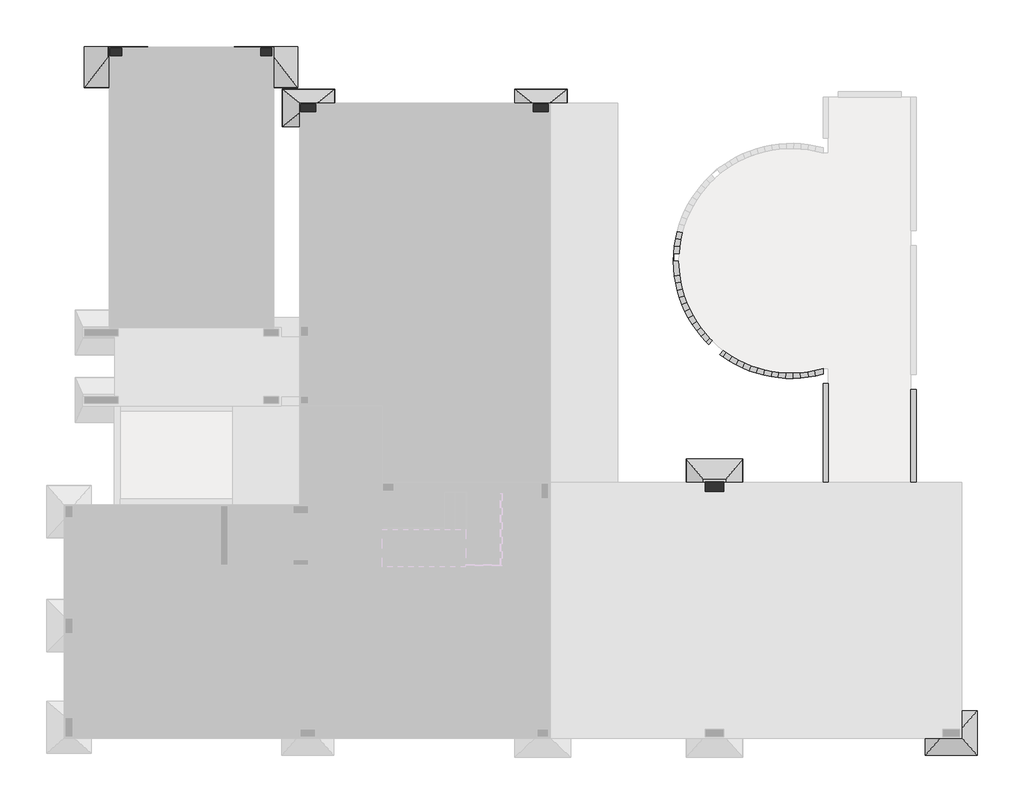
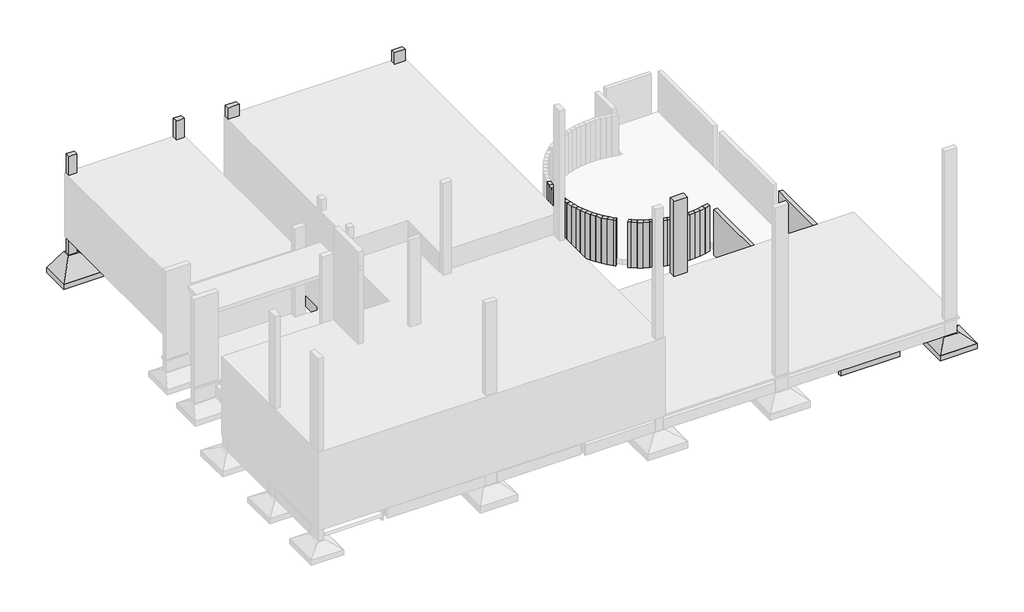
# One storey, part 3 of 4: 37 beams, 7 fasteners, 5 columns.
# Revit data of these elements (continued)
# Type "TQS - Sapata : S13" (continued)
#   EXCXABS = 0.75 m
#   EXCX = 0.00 m
#   DIMY = 1.50 m
#   DIMX = 1.50 m
#   Material estrutural = Concreto - Concreto concretado no local
#   Width = 0
#   Length = 0
# Type "TQS - Sapata : S2"
#   TY = 0.40 m
#   TX = 0.29 m
#   HS = 0.60 m
#   H0 = 0.20 m
#   EXCYABS = 0.85 m
#   EXCY = 0.00 m
#   EXCXABS = 0.145 m
#   EXCX = -0.405 m
#   DIMY = 1.70 m
#   DIMX = 1.10 m
#   Material estrutural = Concreto - Concreto concretado no local
#   Width = 0
#   Length = 0
# Type "TQS - Sapata : S24"
#   TY = 0.60 m
#   TX = 0.29 m
#   HS = 0.50 m
#   H0 = 0.20 m
#   EXCYABS = 0.70 m
#   EXCY = 0.00 m
#   EXCXABS = 0.60 m
#   EXCX = 0.00 m
#   DIMY = 1.40 m
#   DIMX = 1.20 m
#   Material estrutural = Concreto - Concreto concretado no local
#   Width = 0
#   Length = 0
# Type "TQS - Sapata : S3"
#   TY = 0.50 m
#   TX = 0.29 m
#   HS = 0.50 m
#   H0 = 0.20 m
#   EXCYABS = 0.70 m
#   EXCY = 0.00 m
#   EXCXABS = 0.50 m
#   EXCX = 0.00 m
#   DIMY = 1.40 m
#   DIMX = 1.00 m
#   Material estrutural = Concreto - Concreto concretado no local
#   Width = 0
#   Length = 0
# Type "TQS - Sapata : S4"
#   TY = 0.50 m
#   TX = 0.29 m
#   HS = 0.50 m
#   H0 = 0.20 m
#   EXCYABS = 0.70 m
#   EXCY = 0.00 m
#   EXCXABS = 0.50 m
#   EXCX = 0.00 m
#   DIMY = 1.40 m
#   DIMX = 1.00 m
#   Material estrutural = Concreto - Concreto concretado no local
#   Width = 0
#   Length = 0
# Element 1 (IfcBeam, "TQS - Viga retangular : 14.0 x 180.0")
#   Uso = "ESTRUTURA"
#   Titulo = "VP2"
#   Chave = "-984"
#   Tipo Elemento = "Viga"
#   SHA1 = "67BB47F7F07D141E1E461B1B62FFCED57BE49A5E"
#   Revisão = ""
#   Tipo de carga = ""
#   Divisor de flexao = ""
#   Secao = ""
#   Configuracao = ""
#   Angulo (graus) = ""
#   Detalhamento = ""
#   Casos de vento manual = ""
#   Tipo = ""
#   Alcas = ""
#   Furos = ""
#   Pino = ""
#   Distribuicao = ""
#   Solidarizado = ""
#   Solidarizar na montagem = ""
#   Unir com o próximo = ""
#   Grupo pre moldado = ""
#   Verificado = ""
#   Concreto C = ""
#   Taxa de armadura (kgf/m³) = 0
#   Carga (tf/m²) = 0
#   Carga (tf/m) = 0
#   Carga (tf) = 0
#   Altura = 1.80 m
#   Rebaixo = 0.15 m
#   Largura = 0.14 m
#   Distancia a face = 0.00 m
#   Distancia ao eixo = 0.00 m
#   Altura gerber esquerda = 0.00 m
#   Largura gerber esquerda = 0.00 m
#   Altura gerber direita = 0.00 m
#   Largura gerber direita = 0.00 m
#   Resultado de Ensaios fck (MPa) = 0
#   Unique TQS ID = -984
#   Principal = yes
#   Structural Material = none
#   Phase Created = CC_AP/ESTR
# Element 2 (IfcBeam, "TQS - Viga retangular : 14.0 x 180.0")
#   Uso = "ESTRUTURA"
#   Titulo = "VP3"
#   Chave = "-985"
#   Tipo Elemento = "Viga"
#   SHA1 = "1D3F2A738C11C779DD3B877E14C8E10A324E012C"
#   Revisão = ""
#   Tipo de carga = ""
#   Divisor de flexao = ""
#   Secao = ""
#   Configuracao = ""
#   Angulo (graus) = ""
#   Detalhamento = ""
#   Casos de vento manual = ""
#   Tipo = ""
#   Alcas = ""
#   Furos = ""
#   Pino = ""
#   Distribuicao = ""
#   Solidarizado = ""
#   Solidarizar na montagem = ""
#   Unir com o próximo = ""
#   Grupo pre moldado = ""
#   Verificado = ""
#   Concreto C = ""
#   Taxa de armadura (kgf/m³) = 0
#   Carga (tf/m²) = 0
#   Carga (tf/m) = 0
#   Carga (tf) = 0
#   Altura = 1.80 m
#   Rebaixo = 0.15 m
#   Largura = 0.14 m
#   Distancia a face = 0.00 m
#   Distancia ao eixo = 0.00 m
#   Altura gerber esquerda = 0.00 m
#   Largura gerber esquerda = 0.00 m
#   Altura gerber direita = 0.00 m
#   Largura gerber direita = 0.00 m
#   Resultado de Ensaios fck (MPa) = 0
#   Unique TQS ID = -985
#   Principal = yes
#   Structural Material = none
#   Phase Created = CC_AP/ESTR
# Element 3 (IfcBeam, "TQS - Viga retangular : 14.0 x 180.0")
#   Uso = "ESTRUTURA"
#   Titulo = "VP4"
#   Chave = "-987"
#   Tipo Elemento = "Viga"
#   SHA1 = "18E803970E3FF61AE3A7C4B8095E8E40226C0AA9"
#   Revisão = ""
#   Tipo de carga = ""
#   Divisor de flexao = ""
#   Secao = ""
#   Configuracao = ""
#   Angulo (graus) = ""
#   Detalhamento = ""
#   Casos de vento manual = ""
#   Tipo = ""
#   Alcas = ""
#   Furos = ""
#   Pino = ""
#   Distribuicao = ""
#   Solidarizado = ""
#   Solidarizar na montagem = ""
#   Unir com o próximo = ""
#   Grupo pre moldado = ""
#   Verificado = ""
#   Concreto C = ""
#   Taxa de armadura (kgf/m³) = 0
#   Carga (tf/m²) = 0
#   Carga (tf/m) = 0
#   Carga (tf) = 0
#   Altura = 1.80 m
#   Rebaixo = 0.15 m
#   Largura = 0.14 m
#   Distancia a face = 0.00 m
#   Distancia ao eixo = 0.00 m
#   Altura gerber esquerda = 0.00 m
#   Largura gerber esquerda = 0.00 m
#   Altura gerber direita = 0.00 m
#   Largura gerber direita = 0.00 m
#   Resultado de Ensaios fck (MPa) = 0
#   Unique TQS ID = -987
#   Principal = yes
#   Structural Material = none
#   Phase Created = CC_AP/ESTR
# Element 4 (IfcBeam, "TQS - Viga retangular : 14.0 x 180.0")
#   Uso = "ESTRUTURA"
#   Titulo = "VP4"
#   Chave = "-988"
#   Tipo Elemento = "Viga"
#   SHA1 = "B71FF30D7224BC3A2F9C0912C04A339394FFFF18"
#   Revisão = ""
#   Tipo de carga = ""
#   Divisor de flexao = ""
#   Secao = ""
#   Configuracao = ""
#   Angulo (graus) = ""
#   Detalhamento = ""
#   Casos de vento manual = ""
#   Tipo = ""
#   Alcas = ""
#   Furos = ""
#   Pino = ""
#   Distribuicao = ""
#   Solidarizado = ""
#   Solidarizar na montagem = ""
#   Unir com o próximo = ""
#   Grupo pre moldado = ""
#   Verificado = ""
#   Concreto C = ""
#   Taxa de armadura (kgf/m³) = 0
#   Carga (tf/m²) = 0
#   Carga (tf/m) = 0
#   Carga (tf) = 0
#   Altura = 1.80 m
#   Rebaixo = 0.15 m
#   Largura = 0.14 m
#   Distancia a face = 0.00 m
#   Distancia ao eixo = 0.00 m
#   Altura gerber esquerda = 0.00 m
#   Largura gerber esquerda = 0.00 m
#   Altura gerber direita = 0.00 m
#   Largura gerber direita = 0.00 m
#   Resultado de Ensaios fck (MPa) = 0
#   Unique TQS ID = -988
#   Principal = yes
#   Structural Material = none
#   Phase Created = CC_AP/ESTR
# Element 5 (IfcBeam, "TQS - Viga retangular : 14.0 x 180.0")
#   Uso = "ESTRUTURA"
#   Titulo = "VP4"
#   Chave = "-989"
#   Tipo Elemento = "Viga"
#   SHA1 = "E9E1B2FEFAB6FC9E808C50FA3A91823AD53CDAD9"
#   Revisão = ""
#   Tipo de carga = ""
#   Divisor de flexao = ""
#   Secao = ""
#   Configuracao = ""
#   Angulo (graus) = ""
#   Detalhamento = ""
#   Casos de vento manual = ""
#   Tipo = ""
#   Alcas = ""
#   Furos = ""
#   Pino = ""
#   Distribuicao = ""
#   Solidarizado = ""
#   Solidarizar na montagem = ""
#   Unir com o próximo = ""
#   Grupo pre moldado = ""
#   Verificado = ""
#   Concreto C = ""
#   Taxa de armadura (kgf/m³) = 0
#   Carga (tf/m²) = 0
#   Carga (tf/m) = 0
#   Carga (tf) = 0
#   Altura = 1.80 m
#   Rebaixo = 0.15 m
#   Largura = 0.14 m
#   Distancia a face = 0.00 m
#   Distancia ao eixo = 0.00 m
#   Altura gerber esquerda = 0.00 m
#   Largura gerber esquerda = 0.00 m
#   Altura gerber direita = 0.00 m
#   Largura gerber direita = 0.00 m
#   Resultado de Ensaios fck (MPa) = 0
#   Unique TQS ID = -989
#   Principal = yes
#   Structural Material = none
#   Phase Created = CC_AP/ESTR
# Element 6 (IfcBeam, "TQS - Viga retangular : 14.0 x 180.0")
#   Uso = "ESTRUTURA"
#   Titulo = "VP4"
#   Chave = "-990"
#   Tipo Elemento = "Viga"
#   SHA1 = "A4F79934EF83F3B7E9A1E2CD35D009C4681F812D"
#   Revisão = ""
#   Tipo de carga = ""
#   Divisor de flexao = ""
#   Secao = ""
#   Configuracao = ""
#   Angulo (graus) = ""
#   Detalhamento = ""
#   Casos de vento manual = ""
#   Tipo = ""
#   Alcas = ""
#   Furos = ""
#   Pino = ""
#   Distribuicao = ""
#   Solidarizado = ""
#   Solidarizar na montagem = ""
#   Unir com o próximo = ""
#   Grupo pre moldado = ""
#   Verificado = ""
#   Concreto C = ""
#   Taxa de armadura (kgf/m³) = 0
#   Carga (tf/m²) = 0
#   Carga (tf/m) = 0
#   Carga (tf) = 0
#   Altura = 1.80 m
#   Rebaixo = 0.15 m
#   Largura = 0.14 m
#   Distancia a face = 0.00 m
#   Distancia ao eixo = 0.00 m
#   Altura gerber esquerda = 0.00 m
#   Largura gerber esquerda = 0.00 m
#   Altura gerber direita = 0.00 m
#   Largura gerber direita = 0.00 m
#   Resultado de Ensaios fck (MPa) = 0
#   Unique TQS ID = -990
#   Principal = yes
#   Structural Material = none
#   Phase Created = CC_AP/ESTR
# Element 7 (IfcBeam, "TQS - Viga retangular : 14.0 x 180.0")
#   Uso = "ESTRUTURA"
#   Titulo = "VP4"
#   Chave = "-991"
#   Tipo Elemento = "Viga"
#   SHA1 = "59C2882C15F8D77C9BC823B17A9B229971BFE292"
#   Revisão = ""
#   Tipo de carga = ""
#   Divisor de flexao = ""
#   Secao = ""
#   Configuracao = ""
#   Angulo (graus) = ""
#   Detalhamento = ""
#   Casos de vento manual = ""
#   Tipo = ""
#   Alcas = ""
#   Furos = ""
#   Pino = ""
#   Distribuicao = ""
#   Solidarizado = ""
#   Solidarizar na montagem = ""
#   Unir com o próximo = ""
#   Grupo pre moldado = ""
#   Verificado = ""
#   Concreto C = ""
#   Taxa de armadura (kgf/m³) = 0
#   Carga (tf/m²) = 0
#   Carga (tf/m) = 0
#   Carga (tf) = 0
#   Altura = 1.80 m
#   Rebaixo = 0.15 m
#   Largura = 0.14 m
#   Distancia a face = 0.00 m
#   Distancia ao eixo = 0.00 m
#   Altura gerber esquerda = 0.00 m
#   Largura gerber esquerda = 0.00 m
#   Altura gerber direita = 0.00 m
#   Largura gerber direita = 0.00 m
#   Resultado de Ensaios fck (MPa) = 0
#   Unique TQS ID = -991
#   Principal = yes
#   Structural Material = none
#   Phase Created = CC_AP/ESTR
# Element 8 (IfcBeam, "TQS - Viga retangular : 14.0 x 180.0")
#   Uso = "ESTRUTURA"
#   Titulo = "VP4"
#   Chave = "-992"
#   Tipo Elemento = "Viga"
#   SHA1 = "6D985E6B9F5FA1FD140F505980BE925AA5C487F2"
#   Revisão = ""
#   Tipo de carga = ""
#   Divisor de flexao = ""
#   Secao = ""
#   Configuracao = ""
#   Angulo (graus) = ""
#   Detalhamento = ""
#   Casos de vento manual = ""
#   Tipo = ""
#   Alcas = ""
#   Furos = ""
#   Pino = ""
#   Distribuicao = ""
#   Solidarizado = ""
#   Solidarizar na montagem = ""
#   Unir com o próximo = ""
#   Grupo pre moldado = ""
#   Verificado = ""
#   Concreto C = ""
#   Taxa de armadura (kgf/m³) = 0
#   Carga (tf/m²) = 0
#   Carga (tf/m) = 0
#   Carga (tf) = 0
#   Altura = 1.80 m
#   Rebaixo = 0.15 m
#   Largura = 0.14 m
#   Distancia a face = 0.00 m
#   Distancia ao eixo = 0.00 m
#   Altura gerber esquerda = 0.00 m
#   Largura gerber esquerda = 0.00 m
#   Altura gerber direita = 0.00 m
#   Largura gerber direita = 0.00 m
#   Resultado de Ensaios fck (MPa) = 0
#   Unique TQS ID = -992
#   Principal = yes
#   Structural Material = none
#   Phase Created = CC_AP/ESTR
# Element 9 (IfcBeam, "TQS - Viga retangular : 14.0 x 180.0")
#   Uso = "ESTRUTURA"
#   Titulo = "VP4"
#   Chave = "-993"
#   Tipo Elemento = "Viga"
#   SHA1 = "5D4E92287FB362FDFCD64B2B7E6C35302CB92A79"
#   Revisão = ""
#   Tipo de carga = ""
#   Divisor de flexao = ""
#   Secao = ""
#   Configuracao = ""
#   Angulo (graus) = ""
#   Detalhamento = ""
#   Casos de vento manual = ""
#   Tipo = ""
#   Alcas = ""
#   Furos = ""
#   Pino = ""
#   Distribuicao = ""
#   Solidarizado = ""
#   Solidarizar na montagem = ""
#   Unir com o próximo = ""
#   Grupo pre moldado = ""
#   Verificado = ""
#   Concreto C = ""
#   Taxa de armadura (kgf/m³) = 0
#   Carga (tf/m²) = 0
#   Carga (tf/m) = 0
#   Carga (tf) = 0
#   Altura = 1.80 m
#   Rebaixo = 0.15 m
#   Largura = 0.14 m
#   Distancia a face = 0.00 m
#   Distancia ao eixo = 0.00 m
#   Altura gerber esquerda = 0.00 m
#   Largura gerber esquerda = 0.00 m
#   Altura gerber direita = 0.00 m
#   Largura gerber direita = 0.00 m
#   Resultado de Ensaios fck (MPa) = 0
#   Unique TQS ID = -993
#   Principal = yes
#   Structural Material = none
#   Phase Created = CC_AP/ESTR
# Element 10 (IfcBeam, "TQS - Viga retangular : 14.0 x 180.0")
#   Uso = "ESTRUTURA"
#   Titulo = "VP4"
#   Chave = "-994"
#   Tipo Elemento = "Viga"
#   SHA1 = "B241F61C6536B176DF9E3A8727FE075D16BE7057"
#   Revisão = ""
#   Tipo de carga = ""
#   Divisor de flexao = ""
#   Secao = ""
#   Configuracao = ""
#   Angulo (graus) = ""
#   Detalhamento = ""
#   Casos de vento manual = ""
#   Tipo = ""
#   Alcas = ""
#   Furos = ""
#   Pino = ""
#   Distribuicao = ""
#   Solidarizado = ""
#   Solidarizar na montagem = ""
#   Unir com o próximo = ""
#   Grupo pre moldado = ""
#   Verificado = ""
#   Concreto C = ""
#   Taxa de armadura (kgf/m³) = 0
#   Carga (tf/m²) = 0
#   Carga (tf/m) = 0
#   Carga (tf) = 0
#   Altura = 1.80 m
#   Rebaixo = 0.15 m
#   Largura = 0.14 m
#   Distancia a face = 0.00 m
#   Distancia ao eixo = 0.00 m
#   Altura gerber esquerda = 0.00 m
#   Largura gerber esquerda = 0.00 m
#   Altura gerber direita = 0.00 m
#   Largura gerber direita = 0.00 m
#   Resultado de Ensaios fck (MPa) = 0
#   Unique TQS ID = -994
#   Principal = yes
#   Structural Material = none
#   Phase Created = CC_AP/ESTR
# Element 11 (IfcBeam, "TQS - Viga retangular : 14.0 x 180.0")
#   Uso = "ESTRUTURA"
#   Titulo = "VP4"
#   Chave = "-995"
#   Tipo Elemento = "Viga"
#   SHA1 = "79F2E8F443EC2E8CC5B8F506A3E5025E7F953CE7"
#   Revisão = ""
#   Tipo de carga = ""
#   Divisor de flexao = ""
#   Secao = ""
#   Configuracao = ""
#   Angulo (graus) = ""
#   Detalhamento = ""
#   Casos de vento manual = ""
#   Tipo = ""
#   Alcas = ""
#   Furos = ""
#   Pino = ""
#   Distribuicao = ""
#   Solidarizado = ""
#   Solidarizar na montagem = ""
#   Unir com o próximo = ""
#   Grupo pre moldado = ""
#   Verificado = ""
#   Concreto C = ""
#   Taxa de armadura (kgf/m³) = 0
#   Carga (tf/m²) = 0
#   Carga (tf/m) = 0
#   Carga (tf) = 0
#   Altura = 1.80 m
#   Rebaixo = 0.15 m
#   Largura = 0.14 m
#   Distancia a face = 0.00 m
#   Distancia ao eixo = 0.00 m
#   Altura gerber esquerda = 0.00 m
#   Largura gerber esquerda = 0.00 m
#   Altura gerber direita = 0.00 m
#   Largura gerber direita = 0.00 m
#   Resultado de Ensaios fck (MPa) = 0
#   Unique TQS ID = -995
#   Principal = yes
#   Structural Material = none
#   Phase Created = CC_AP/ESTR
# Element 12 (IfcBeam, "TQS - Viga retangular : 14.0 x 180.0")
#   Uso = "ESTRUTURA"
#   Titulo = "VP4"
#   Chave = "-996"
#   Tipo Elemento = "Viga"
#   SHA1 = "EC69CF733B6B75DD72A616518C986B1D4EC6373A"
#   Revisão = ""
#   Tipo de carga = ""
#   Divisor de flexao = ""
#   Secao = ""
#   Configuracao = ""
#   Angulo (graus) = ""
#   Detalhamento = ""
#   Casos de vento manual = ""
#   Tipo = ""
#   Alcas = ""
#   Furos = ""
#   Pino = ""
#   Distribuicao = ""
#   Solidarizado = ""
#   Solidarizar na montagem = ""
#   Unir com o próximo = ""
#   Grupo pre moldado = ""
#   Verificado = ""
#   Concreto C = ""
#   Taxa de armadura (kgf/m³) = 0
#   Carga (tf/m²) = 0
#   Carga (tf/m) = 0
#   Carga (tf) = 0
#   Altura = 1.80 m
#   Rebaixo = 0.15 m
#   Largura = 0.14 m
#   Distancia a face = 0.00 m
#   Distancia ao eixo = 0.00 m
#   Altura gerber esquerda = 0.00 m
#   Largura gerber esquerda = 0.00 m
#   Altura gerber direita = 0.00 m
#   Largura gerber direita = 0.00 m
#   Resultado de Ensaios fck (MPa) = 0
#   Unique TQS ID = -996
#   Principal = yes
#   Structural Material = none
#   Phase Created = CC_AP/ESTR
# Element 13 (IfcBeam, "TQS - Viga retangular : 14.0 x 180.0")
#   Uso = "ESTRUTURA"
#   Titulo = "VP4"
#   Chave = "-997"
#   Tipo Elemento = "Viga"
#   SHA1 = "A94BB0AB94C95055560F49AF3BCE408F9E38B8C0"
#   Revisão = ""
#   Tipo de carga = ""
#   Divisor de flexao = ""
#   Secao = ""
#   Configuracao = ""
#   Angulo (graus) = ""
#   Detalhamento = ""
#   Casos de vento manual = ""
#   Tipo = ""
#   Alcas = ""
#   Furos = ""
#   Pino = ""
#   Distribuicao = ""
#   Solidarizado = ""
#   Solidarizar na montagem = ""
#   Unir com o próximo = ""
#   Grupo pre moldado = ""
#   Verificado = ""
#   Concreto C = ""
#   Taxa de armadura (kgf/m³) = 0
#   Carga (tf/m²) = 0
#   Carga (tf/m) = 0
#   Carga (tf) = 0
#   Altura = 1.80 m
#   Rebaixo = 0.15 m
#   Largura = 0.14 m
#   Distancia a face = 0.00 m
#   Distancia ao eixo = 0.00 m
#   Altura gerber esquerda = 0.00 m
#   Largura gerber esquerda = 0.00 m
#   Altura gerber direita = 0.00 m
#   Largura gerber direita = 0.00 m
#   Resultado de Ensaios fck (MPa) = 0
#   Unique TQS ID = -997
#   Principal = yes
#   Structural Material = none
#   Phase Created = CC_AP/ESTR
# Element 14 (IfcBeam, "TQS - Viga retangular : 14.0 x 180.0")
#   Uso = "ESTRUTURA"
#   Titulo = "VP4"
#   Chave = "-998"
#   Tipo Elemento = "Viga"
#   SHA1 = "6378FB8D39603434150BF0AD569D703CFB80FE5F"
#   Revisão = ""
#   Tipo de carga = ""
#   Divisor de flexao = ""
#   Secao = ""
#   Configuracao = ""
#   Angulo (graus) = ""
#   Detalhamento = ""
#   Casos de vento manual = ""
#   Tipo = ""
#   Alcas = ""
#   Furos = ""
#   Pino = ""
#   Distribuicao = ""
#   Solidarizado = ""
#   Solidarizar na montagem = ""
#   Unir com o próximo = ""
#   Grupo pre moldado = ""
#   Verificado = ""
#   Concreto C = ""
#   Taxa de armadura (kgf/m³) = 0
#   Carga (tf/m²) = 0
#   Carga (tf/m) = 0
#   Carga (tf) = 0
#   Altura = 1.80 m
#   Rebaixo = 0.15 m
#   Largura = 0.14 m
#   Distancia a face = 0.00 m
#   Distancia ao eixo = 0.00 m
#   Altura gerber esquerda = 0.00 m
#   Largura gerber esquerda = 0.00 m
#   Altura gerber direita = 0.00 m
#   Largura gerber direita = 0.00 m
#   Resultado de Ensaios fck (MPa) = 0
#   Unique TQS ID = -998
#   Principal = yes
#   Structural Material = none
#   Phase Created = CC_AP/ESTR
# Element 15 (IfcBeam, "TQS - Viga retangular : 14.0 x 180.0")
#   Uso = "ESTRUTURA"
#   Titulo = "VP4"
#   Chave = "-999"
#   Tipo Elemento = "Viga"
#   SHA1 = "2B4C78D211D826E735DAAC0C825AB5B97130EBCE"
#   Revisão = ""
#   Tipo de carga = ""
#   Divisor de flexao = ""
#   Secao = ""
#   Configuracao = ""
#   Angulo (graus) = ""
#   Detalhamento = ""
#   Casos de vento manual = ""
#   Tipo = ""
#   Alcas = ""
#   Furos = ""
#   Pino = ""
#   Distribuicao = ""
#   Solidarizado = ""
#   Solidarizar na montagem = ""
#   Unir com o próximo = ""
#   Grupo pre moldado = ""
#   Verificado = ""
#   Concreto C = ""
#   Taxa de armadura (kgf/m³) = 0
#   Carga (tf/m²) = 0
#   Carga (tf/m) = 0
#   Carga (tf) = 0
#   Altura = 1.80 m
#   Rebaixo = 0.15 m
#   Largura = 0.14 m
#   Distancia a face = 0.00 m
#   Distancia ao eixo = 0.00 m
#   Altura gerber esquerda = 0.00 m
#   Largura gerber esquerda = 0.00 m
#   Altura gerber direita = 0.00 m
#   Largura gerber direita = 0.00 m
#   Resultado de Ensaios fck (MPa) = 0
#   Unique TQS ID = -999
#   Principal = yes
#   Structural Material = none
#   Phase Created = CC_AP/ESTR
# Element 16 (IfcBeam, "TQS - Viga retangular : 14.0 x 180.0")
#   Uso = "ESTRUTURA"
#   Titulo = "VP4"
#   Chave = "-1000"
#   Tipo Elemento = "Viga"
#   SHA1 = "DD50D292EAFD20D7EF85643CCD075ACF91033CA0"
#   Revisão = ""
#   Tipo de carga = ""
#   Divisor de flexao = ""
#   Secao = ""
#   Configuracao = ""
#   Angulo (graus) = ""
#   Detalhamento = ""
#   Casos de vento manual = ""
#   Tipo = ""
#   Alcas = ""
#   Furos = ""
#   Pino = ""
#   Distribuicao = ""
#   Solidarizado = ""
#   Solidarizar na montagem = ""
#   Unir com o próximo = ""
#   Grupo pre moldado = ""
#   Verificado = ""
#   Concreto C = ""
#   Taxa de armadura (kgf/m³) = 0
#   Carga (tf/m²) = 0
#   Carga (tf/m) = 0
#   Carga (tf) = 0
#   Altura = 1.80 m
#   Rebaixo = 0.15 m
#   Largura = 0.14 m
#   Distancia a face = 0.00 m
#   Distancia ao eixo = 0.00 m
#   Altura gerber esquerda = 0.00 m
#   Largura gerber esquerda = 0.00 m
#   Altura gerber direita = 0.00 m
#   Largura gerber direita = 0.00 m
#   Resultado de Ensaios fck (MPa) = 0
#   Unique TQS ID = -1000
#   Principal = yes
#   Structural Material = none
#   Phase Created = CC_AP/ESTR
# Element 17 (IfcBeam, "TQS - Viga retangular : 14.0 x 180.0")
#   Uso = "ESTRUTURA"
#   Titulo = "VP4"
#   Chave = "-1001"
#   Tipo Elemento = "Viga"
#   SHA1 = "17AE169FA700E73A155B49B14AA872A50BD18F4B"
#   Revisão = ""
#   Tipo de carga = ""
#   Divisor de flexao = ""
#   Secao = ""
#   Configuracao = ""
#   Angulo (graus) = ""
#   Detalhamento = ""
#   Casos de vento manual = ""
#   Tipo = ""
#   Alcas = ""
#   Furos = ""
#   Pino = ""
#   Distribuicao = ""
#   Solidarizado = ""
#   Solidarizar na montagem = ""
#   Unir com o próximo = ""
#   Grupo pre moldado = ""
#   Verificado = ""
#   Concreto C = ""
#   Taxa de armadura (kgf/m³) = 0
#   Carga (tf/m²) = 0
#   Carga (tf/m) = 0
#   Carga (tf) = 0
#   Altura = 1.80 m
#   Rebaixo = 0.15 m
#   Largura = 0.14 m
#   Distancia a face = 0.00 m
#   Distancia ao eixo = 0.00 m
#   Altura gerber esquerda = 0.00 m
#   Largura gerber esquerda = 0.00 m
#   Altura gerber direita = 0.00 m
#   Largura gerber direita = 0.00 m
#   Resultado de Ensaios fck (MPa) = 0
#   Unique TQS ID = -1001
#   Principal = yes
#   Structural Material = none
#   Phase Created = CC_AP/ESTR
# Element 18 (IfcBeam, "TQS - Viga retangular : 14.0 x 180.0")
#   Uso = "ESTRUTURA"
#   Titulo = "VP5"
#   Chave = "-1002"
#   Tipo Elemento = "Viga"
#   SHA1 = "4C02C5B53EDBB34F44F4EAF2E9EE20AD89CC6C79"
#   Revisão = ""
#   Tipo de carga = ""
#   Divisor de flexao = ""
#   Secao = ""
#   Configuracao = ""
#   Angulo (graus) = ""
#   Detalhamento = ""
#   Casos de vento manual = ""
#   Tipo = ""
#   Alcas = ""
#   Furos = ""
#   Pino = ""
#   Distribuicao = ""
#   Solidarizado = ""
#   Solidarizar na montagem = ""
#   Unir com o próximo = ""
#   Grupo pre moldado = ""
#   Verificado = ""
#   Concreto C = ""
#   Taxa de armadura (kgf/m³) = 0
#   Carga (tf/m²) = 0
#   Carga (tf/m) = 0
#   Carga (tf) = 0
#   Altura = 1.80 m
#   Rebaixo = 0.15 m
#   Largura = 0.14 m
#   Distancia a face = 0.00 m
#   Distancia ao eixo = 0.00 m
#   Altura gerber esquerda = 0.00 m
#   Largura gerber esquerda = 0.00 m
#   Altura gerber direita = 0.00 m
#   Largura gerber direita = 0.00 m
#   Resultado de Ensaios fck (MPa) = 0
#   Unique TQS ID = -1002
#   Principal = yes
#   Structural Material = none
#   Phase Created = CC_AP/ESTR
# Element 19 (IfcBeam, "TQS - Viga retangular : 14.0 x 180.0")
#   Uso = "ESTRUTURA"
#   Titulo = "VP5"
#   Chave = "-1003"
#   Tipo Elemento = "Viga"
#   SHA1 = "4CC80C174DC5A33A4959CFE9988141447D2CA55C"
#   Revisão = ""
#   Tipo de carga = ""
#   Divisor de flexao = ""
#   Secao = ""
#   Configuracao = ""
#   Angulo (graus) = ""
#   Detalhamento = ""
#   Casos de vento manual = ""
#   Tipo = ""
#   Alcas = ""
#   Furos = ""
#   Pino = ""
#   Distribuicao = ""
#   Solidarizado = ""
#   Solidarizar na montagem = ""
#   Unir com o próximo = ""
#   Grupo pre moldado = ""
#   Verificado = ""
#   Concreto C = ""
#   Taxa de armadura (kgf/m³) = 0
#   Carga (tf/m²) = 0
#   Carga (tf/m) = 0
#   Carga (tf) = 0
#   Altura = 1.80 m
#   Rebaixo = 0.15 m
#   Largura = 0.14 m
#   Distancia a face = 0.00 m
#   Distancia ao eixo = 0.00 m
#   Altura gerber esquerda = 0.00 m
#   Largura gerber esquerda = 0.00 m
#   Altura gerber direita = 0.00 m
#   Largura gerber direita = 0.00 m
#   Resultado de Ensaios fck (MPa) = 0
#   Unique TQS ID = -1003
#   Principal = yes
#   Structural Material = none
#   Phase Created = CC_AP/ESTR
# Element 20 (IfcBeam, "TQS - Viga retangular : 14.0 x 180.0")
#   Uso = "ESTRUTURA"
#   Titulo = "VP5"
#   Chave = "-1004"
#   Tipo Elemento = "Viga"
#   SHA1 = "B47BB11AE5BEE4DA1AC1C982C2FC48DC4A5ED7AF"
#   Revisão = ""
#   Tipo de carga = ""
#   Divisor de flexao = ""
#   Secao = ""
#   Configuracao = ""
#   Angulo (graus) = ""
#   Detalhamento = ""
#   Casos de vento manual = ""
#   Tipo = ""
#   Alcas = ""
#   Furos = ""
#   Pino = ""
#   Distribuicao = ""
#   Solidarizado = ""
#   Solidarizar na montagem = ""
#   Unir com o próximo = ""
#   Grupo pre moldado = ""
#   Verificado = ""
#   Concreto C = ""
#   Taxa de armadura (kgf/m³) = 0
#   Carga (tf/m²) = 0
#   Carga (tf/m) = 0
#   Carga (tf) = 0
#   Altura = 1.80 m
#   Rebaixo = 0.15 m
#   Largura = 0.14 m
#   Distancia a face = 0.00 m
#   Distancia ao eixo = 0.00 m
#   Altura gerber esquerda = 0.00 m
#   Largura gerber esquerda = 0.00 m
#   Altura gerber direita = 0.00 m
#   Largura gerber direita = 0.00 m
#   Resultado de Ensaios fck (MPa) = 0
#   Unique TQS ID = -1004
#   Principal = yes
#   Structural Material = none
#   Phase Created = CC_AP/ESTR
# Element 21 (IfcBeam, "TQS - Viga retangular : 14.0 x 180.0")
#   Uso = "ESTRUTURA"
#   Titulo = "VP5"
#   Chave = "-1005"
#   Tipo Elemento = "Viga"
#   SHA1 = "D99F413EAFADC372BC776638DB624CCF8BA82056"
#   Revisão = ""
#   Tipo de carga = ""
#   Divisor de flexao = ""
#   Secao = ""
#   Configuracao = ""
#   Angulo (graus) = ""
#   Detalhamento = ""
#   Casos de vento manual = ""
#   Tipo = ""
#   Alcas = ""
#   Furos = ""
#   Pino = ""
#   Distribuicao = ""
#   Solidarizado = ""
#   Solidarizar na montagem = ""
#   Unir com o próximo = ""
#   Grupo pre moldado = ""
#   Verificado = ""
#   Concreto C = ""
#   Taxa de armadura (kgf/m³) = 0
#   Carga (tf/m²) = 0
#   Carga (tf/m) = 0
#   Carga (tf) = 0
#   Altura = 1.80 m
#   Rebaixo = 0.15 m
#   Largura = 0.14 m
#   Distancia a face = 0.00 m
#   Distancia ao eixo = 0.00 m
#   Altura gerber esquerda = 0.00 m
#   Largura gerber esquerda = 0.00 m
#   Altura gerber direita = 0.00 m
#   Largura gerber direita = 0.00 m
#   Resultado de Ensaios fck (MPa) = 0
#   Unique TQS ID = -1005
#   Principal = yes
#   Structural Material = none
#   Phase Created = CC_AP/ESTR
# Element 22 (IfcBeam, "TQS - Viga retangular : 14.0 x 180.0")
#   Uso = "ESTRUTURA"
#   Titulo = "VP5"
#   Chave = "-1006"
#   Tipo Elemento = "Viga"
#   SHA1 = "45441B0255AB8A379653287FCCEE7CF9E9C67E02"
#   Revisão = ""
#   Tipo de carga = ""
#   Divisor de flexao = ""
#   Secao = ""
#   Configuracao = ""
#   Angulo (graus) = ""
#   Detalhamento = ""
#   Casos de vento manual = ""
#   Tipo = ""
#   Alcas = ""
#   Furos = ""
#   Pino = ""
#   Distribuicao = ""
#   Solidarizado = ""
#   Solidarizar na montagem = ""
#   Unir com o próximo = ""
#   Grupo pre moldado = ""
#   Verificado = ""
#   Concreto C = ""
#   Taxa de armadura (kgf/m³) = 0
#   Carga (tf/m²) = 0
#   Carga (tf/m) = 0
#   Carga (tf) = 0
#   Altura = 1.80 m
#   Rebaixo = 0.15 m
#   Largura = 0.14 m
#   Distancia a face = 0.00 m
#   Distancia ao eixo = 0.00 m
#   Altura gerber esquerda = 0.00 m
#   Largura gerber esquerda = 0.00 m
#   Altura gerber direita = 0.00 m
#   Largura gerber direita = 0.00 m
#   Resultado de Ensaios fck (MPa) = 0
#   Unique TQS ID = -1006
#   Principal = yes
#   Structural Material = none
#   Phase Created = CC_AP/ESTR
# Element 23 (IfcBeam, "TQS - Viga retangular : 14.0 x 180.0")
#   Uso = "ESTRUTURA"
#   Titulo = "VP5"
#   Chave = "-1007"
#   Tipo Elemento = "Viga"
#   SHA1 = "67D8F0B72EA773B01EE7283A9BF6FD7CCC373B16"
#   Revisão = ""
#   Tipo de carga = ""
#   Divisor de flexao = ""
#   Secao = ""
#   Configuracao = ""
#   Angulo (graus) = ""
#   Detalhamento = ""
#   Casos de vento manual = ""
#   Tipo = ""
#   Alcas = ""
#   Furos = ""
#   Pino = ""
#   Distribuicao = ""
#   Solidarizado = ""
#   Solidarizar na montagem = ""
#   Unir com o próximo = ""
#   Grupo pre moldado = ""
#   Verificado = ""
#   Concreto C = ""
#   Taxa de armadura (kgf/m³) = 0
#   Carga (tf/m²) = 0
#   Carga (tf/m) = 0
#   Carga (tf) = 0
#   Altura = 1.80 m
#   Rebaixo = 0.15 m
#   Largura = 0.14 m
#   Distancia a face = 0.00 m
#   Distancia ao eixo = 0.00 m
#   Altura gerber esquerda = 0.00 m
#   Largura gerber esquerda = 0.00 m
#   Altura gerber direita = 0.00 m
#   Largura gerber direita = 0.00 m
#   Resultado de Ensaios fck (MPa) = 0
#   Unique TQS ID = -1007
#   Principal = yes
#   Structural Material = none
#   Phase Created = CC_AP/ESTR
# Element 24 (IfcBeam, "TQS - Viga retangular : 14.0 x 180.0")
#   Uso = "ESTRUTURA"
#   Titulo = "VP5"
#   Chave = "-1008"
#   Tipo Elemento = "Viga"
#   SHA1 = "97D86C514C265A9FC3405D75886B30F1FDE07F5F"
#   Revisão = ""
#   Tipo de carga = ""
#   Divisor de flexao = ""
#   Secao = ""
#   Configuracao = ""
#   Angulo (graus) = ""
#   Detalhamento = ""
#   Casos de vento manual = ""
#   Tipo = ""
#   Alcas = ""
#   Furos = ""
#   Pino = ""
#   Distribuicao = ""
#   Solidarizado = ""
#   Solidarizar na montagem = ""
#   Unir com o próximo = ""
#   Grupo pre moldado = ""
#   Verificado = ""
#   Concreto C = ""
#   Taxa de armadura (kgf/m³) = 0
#   Carga (tf/m²) = 0
#   Carga (tf/m) = 0
#   Carga (tf) = 0
#   Altura = 1.80 m
#   Rebaixo = 0.15 m
#   Largura = 0.14 m
#   Distancia a face = 0.00 m
#   Distancia ao eixo = 0.00 m
#   Altura gerber esquerda = 0.00 m
#   Largura gerber esquerda = 0.00 m
#   Altura gerber direita = 0.00 m
#   Largura gerber direita = 0.00 m
#   Resultado de Ensaios fck (MPa) = 0
#   Unique TQS ID = -1008
#   Principal = yes
#   Structural Material = none
#   Phase Created = CC_AP/ESTR
# Element 25 (IfcBeam, "TQS - Viga retangular : 14.0 x 180.0")
#   Uso = "ESTRUTURA"
#   Titulo = "VP5"
#   Chave = "-1009"
#   Tipo Elemento = "Viga"
#   SHA1 = "E11E876F0FB2670C71699C66FE517DB49DCFCCF5"
#   Revisão = ""
#   Tipo de carga = ""
#   Divisor de flexao = ""
#   Secao = ""
#   Configuracao = ""
#   Angulo (graus) = ""
#   Detalhamento = ""
#   Casos de vento manual = ""
#   Tipo = ""
#   Alcas = ""
#   Furos = ""
#   Pino = ""
#   Distribuicao = ""
#   Solidarizado = ""
#   Solidarizar na montagem = ""
#   Unir com o próximo = ""
#   Grupo pre moldado = ""
#   Verificado = ""
#   Concreto C = ""
#   Taxa de armadura (kgf/m³) = 0
#   Carga (tf/m²) = 0
#   Carga (tf/m) = 0
#   Carga (tf) = 0
#   Altura = 1.80 m
#   Rebaixo = 0.15 m
#   Largura = 0.14 m
#   Distancia a face = 0.00 m
#   Distancia ao eixo = 0.00 m
#   Altura gerber esquerda = 0.00 m
#   Largura gerber esquerda = 0.00 m
#   Altura gerber direita = 0.00 m
#   Largura gerber direita = 0.00 m
#   Resultado de Ensaios fck (MPa) = 0
#   Unique TQS ID = -1009
#   Principal = yes
#   Structural Material = none
#   Phase Created = CC_AP/ESTR
# Element 26 (IfcBeam, "TQS - Viga retangular : 14.0 x 180.0")
#   Uso = "ESTRUTURA"
#   Titulo = "VP5"
#   Chave = "-1010"
#   Tipo Elemento = "Viga"
#   SHA1 = "B2FE66282E83D533D9B7EA94ACB770D2301BAEA7"
#   Revisão = ""
#   Tipo de carga = ""
#   Divisor de flexao = ""
#   Secao = ""
#   Configuracao = ""
#   Angulo (graus) = ""
#   Detalhamento = ""
#   Casos de vento manual = ""
#   Tipo = ""
#   Alcas = ""
#   Furos = ""
#   Pino = ""
#   Distribuicao = ""
#   Solidarizado = ""
#   Solidarizar na montagem = ""
#   Unir com o próximo = ""
#   Grupo pre moldado = ""
#   Verificado = ""
#   Concreto C = ""
#   Taxa de armadura (kgf/m³) = 0
#   Carga (tf/m²) = 0
#   Carga (tf/m) = 0
#   Carga (tf) = 0
#   Altura = 1.80 m
#   Rebaixo = 0.15 m
#   Largura = 0.14 m
#   Distancia a face = 0.00 m
#   Distancia ao eixo = 0.00 m
#   Altura gerber esquerda = 0.00 m
#   Largura gerber esquerda = 0.00 m
#   Altura gerber direita = 0.00 m
#   Largura gerber direita = 0.00 m
#   Resultado de Ensaios fck (MPa) = 0
#   Unique TQS ID = -1010
#   Principal = yes
#   Structural Material = none
#   Phase Created = CC_AP/ESTR
# Element 27 (IfcBeam, "TQS - Viga retangular : 14.0 x 180.0")
#   Uso = "ESTRUTURA"
#   Titulo = "VP5"
#   Chave = "-1011"
#   Tipo Elemento = "Viga"
#   SHA1 = "B326764AED5F8992A99CC84B56FBCB9058379F2E"
#   Revisão = ""
#   Tipo de carga = ""
#   Divisor de flexao = ""
#   Secao = ""
#   Configuracao = ""
#   Angulo (graus) = ""
#   Detalhamento = ""
#   Casos de vento manual = ""
#   Tipo = ""
#   Alcas = ""
#   Furos = ""
#   Pino = ""
#   Distribuicao = ""
#   Solidarizado = ""
#   Solidarizar na montagem = ""
#   Unir com o próximo = ""
#   Grupo pre moldado = ""
#   Verificado = ""
#   Concreto C = ""
#   Taxa de armadura (kgf/m³) = 0
#   Carga (tf/m²) = 0
#   Carga (tf/m) = 0
#   Carga (tf) = 0
#   Altura = 1.80 m
#   Rebaixo = 0.15 m
#   Largura = 0.14 m
#   Distancia a face = 0.00 m
#   Distancia ao eixo = 0.00 m
#   Altura gerber esquerda = 0.00 m
#   Largura gerber esquerda = 0.00 m
#   Altura gerber direita = 0.00 m
#   Largura gerber direita = 0.00 m
#   Resultado de Ensaios fck (MPa) = 0
#   Unique TQS ID = -1011
#   Principal = yes
#   Structural Material = none
#   Phase Created = CC_AP/ESTR
# Element 28 (IfcBeam, "TQS - Viga retangular : 14.0 x 180.0")
#   Uso = "ESTRUTURA"
#   Titulo = "VP5"
#   Chave = "-1012"
#   Tipo Elemento = "Viga"
#   SHA1 = "ADF8088E05543C33AE80BF92F8ECBD3B445E80A1"
#   Revisão = ""
#   Tipo de carga = ""
#   Divisor de flexao = ""
#   Secao = ""
#   Configuracao = ""
#   Angulo (graus) = ""
#   Detalhamento = ""
#   Casos de vento manual = ""
#   Tipo = ""
#   Alcas = ""
#   Furos = ""
#   Pino = ""
#   Distribuicao = ""
#   Solidarizado = ""
#   Solidarizar na montagem = ""
#   Unir com o próximo = ""
#   Grupo pre moldado = ""
#   Verificado = ""
#   Concreto C = ""
#   Taxa de armadura (kgf/m³) = 0
#   Carga (tf/m²) = 0
#   Carga (tf/m) = 0
#   Carga (tf) = 0
#   Altura = 1.80 m
#   Rebaixo = 0.15 m
#   Largura = 0.14 m
#   Distancia a face = 0.00 m
#   Distancia ao eixo = 0.00 m
#   Altura gerber esquerda = 0.00 m
#   Largura gerber esquerda = 0.00 m
#   Altura gerber direita = 0.00 m
#   Largura gerber direita = 0.00 m
#   Resultado de Ensaios fck (MPa) = 0
#   Unique TQS ID = -1012
#   Principal = yes
#   Structural Material = none
#   Phase Created = CC_AP/ESTR
# Element 29 (IfcBeam, "TQS - Viga retangular : 14.0 x 180.0")
#   Uso = "ESTRUTURA"
#   Titulo = "VP5"
#   Chave = "-1013"
#   Tipo Elemento = "Viga"
#   SHA1 = "F629BC16B5B7CEFABB33876C532E6A3B47A757C7"
#   Revisão = ""
#   Tipo de carga = ""
#   Divisor de flexao = ""
#   Secao = ""
#   Configuracao = ""
#   Angulo (graus) = ""
#   Detalhamento = ""
#   Casos de vento manual = ""
#   Tipo = ""
#   Alcas = ""
#   Furos = ""
#   Pino = ""
#   Distribuicao = ""
#   Solidarizado = ""
#   Solidarizar na montagem = ""
#   Unir com o próximo = ""
#   Grupo pre moldado = ""
#   Verificado = ""
#   Concreto C = ""
#   Taxa de armadura (kgf/m³) = 0
#   Carga (tf/m²) = 0
#   Carga (tf/m) = 0
#   Carga (tf) = 0
#   Altura = 1.80 m
#   Rebaixo = 0.15 m
#   Largura = 0.14 m
#   Distancia a face = 0.00 m
#   Distancia ao eixo = 0.00 m
#   Altura gerber esquerda = 0.00 m
#   Largura gerber esquerda = 0.00 m
#   Altura gerber direita = 0.00 m
#   Largura gerber direita = 0.00 m
#   Resultado de Ensaios fck (MPa) = 0
#   Unique TQS ID = -1013
#   Principal = yes
#   Structural Material = none
#   Phase Created = CC_AP/ESTR
# Element 30 (IfcBeam, "TQS - Viga retangular : 14.0 x 180.0")
#   Uso = "ESTRUTURA"
#   Titulo = "VP6"
#   Chave = "-1014"
#   Tipo Elemento = "Viga"
#   SHA1 = "803FE0467B8784052CD3520716E944CE5BCDE54C"
#   Revisão = ""
#   Tipo de carga = ""
#   Divisor de flexao = ""
#   Secao = ""
#   Configuracao = ""
#   Angulo (graus) = ""
#   Detalhamento = ""
#   Casos de vento manual = ""
#   Tipo = ""
#   Alcas = ""
#   Furos = ""
#   Pino = ""
#   Distribuicao = ""
#   Solidarizado = ""
#   Solidarizar na montagem = ""
#   Unir com o próximo = ""
#   Grupo pre moldado = ""
#   Verificado = ""
#   Concreto C = ""
#   Taxa de armadura (kgf/m³) = 0
#   Carga (tf/m²) = 0
#   Carga (tf/m) = 0
#   Carga (tf) = 0
#   Altura = 1.80 m
#   Rebaixo = 0.15 m
#   Largura = 0.14 m
#   Distancia a face = 0.00 m
#   Distancia ao eixo = 0.00 m
#   Altura gerber esquerda = 0.00 m
#   Largura gerber esquerda = 0.00 m
#   Altura gerber direita = 0.00 m
#   Largura gerber direita = 0.00 m
#   Resultado de Ensaios fck (MPa) = 0
#   Unique TQS ID = -1014
#   Principal = yes
#   Structural Material = none
#   Phase Created = CC_AP/ESTR
# Element 31 (IfcBeam, "TQS - Viga retangular : 14.0 x 180.0")
#   Uso = "ESTRUTURA"
#   Titulo = "VP6"
#   Chave = "-1015"
#   Tipo Elemento = "Viga"
#   SHA1 = "4E9806910888EA421A8E9B5F41FC3E19263D6A9E"
#   Revisão = ""
#   Tipo de carga = ""
#   Divisor de flexao = ""
#   Secao = ""
#   Configuracao = ""
#   Angulo (graus) = ""
#   Detalhamento = ""
#   Casos de vento manual = ""
#   Tipo = ""
#   Alcas = ""
#   Furos = ""
#   Pino = ""
#   Distribuicao = ""
#   Solidarizado = ""
#   Solidarizar na montagem = ""
#   Unir com o próximo = ""
#   Grupo pre moldado = ""
#   Verificado = ""
#   Concreto C = ""
#   Taxa de armadura (kgf/m³) = 0
#   Carga (tf/m²) = 0
#   Carga (tf/m) = 0
#   Carga (tf) = 0
#   Altura = 1.80 m
#   Rebaixo = 0.15 m
#   Largura = 0.14 m
#   Distancia a face = 0.00 m
#   Distancia ao eixo = 0.00 m
#   Altura gerber esquerda = 0.00 m
#   Largura gerber esquerda = 0.00 m
#   Altura gerber direita = 0.00 m
#   Largura gerber direita = 0.00 m
#   Resultado de Ensaios fck (MPa) = 0
#   Unique TQS ID = -1015
#   Principal = yes
#   Structural Material = none
#   Phase Created = CC_AP/ESTR
# Element 32 (IfcBeam, "TQS - Viga retangular : 14.0 x 180.0")
#   Uso = "ESTRUTURA"
#   Titulo = "VP6"
#   Chave = "-1016"
#   Tipo Elemento = "Viga"
#   SHA1 = "01F1283C1B0C380DFDB901244E097327FB4B1C7E"
#   Revisão = ""
#   Tipo de carga = ""
#   Divisor de flexao = ""
#   Secao = ""
#   Configuracao = ""
#   Angulo (graus) = ""
#   Detalhamento = ""
#   Casos de vento manual = ""
#   Tipo = ""
#   Alcas = ""
#   Furos = ""
#   Pino = ""
#   Distribuicao = ""
#   Solidarizado = ""
#   Solidarizar na montagem = ""
#   Unir com o próximo = ""
#   Grupo pre moldado = ""
#   Verificado = ""
#   Concreto C = ""
#   Taxa de armadura (kgf/m³) = 0
#   Carga (tf/m²) = 0
#   Carga (tf/m) = 0
#   Carga (tf) = 0
#   Altura = 1.80 m
#   Rebaixo = 0.15 m
#   Largura = 0.14 m
#   Distancia a face = 0.00 m
#   Distancia ao eixo = 0.00 m
#   Altura gerber esquerda = 0.00 m
#   Largura gerber esquerda = 0.00 m
#   Altura gerber direita = 0.00 m
#   Largura gerber direita = 0.00 m
#   Resultado de Ensaios fck (MPa) = 0
#   Unique TQS ID = -1016
#   Principal = yes
#   Structural Material = none
#   Phase Created = CC_AP/ESTR
# Element 33 (IfcBeam, "TQS - Viga retangular : 14.0 x 180.0")
#   Uso = "ESTRUTURA"
#   Titulo = "VP9"
#   Chave = "-1042"
#   Tipo Elemento = "Viga"
#   SHA1 = "A33BDDD61DCA14C8FF84777102E10ABF9273446C"
#   Revisão = ""
#   Tipo de carga = ""
#   Divisor de flexao = ""
#   Secao = ""
#   Configuracao = ""
#   Angulo (graus) = ""
#   Detalhamento = ""
#   Casos de vento manual = ""
#   Tipo = ""
#   Alcas = ""
#   Furos = ""
#   Pino = ""
#   Distribuicao = ""
#   Solidarizado = ""
#   Solidarizar na montagem = ""
#   Unir com o próximo = ""
#   Grupo pre moldado = ""
#   Verificado = ""
#   Concreto C = ""
#   Taxa de armadura (kgf/m³) = 0
#   Carga (tf/m²) = 0
#   Carga (tf/m) = 0
#   Carga (tf) = 0
#   Altura = 1.80 m
#   Rebaixo = 0.15 m
#   Largura = 0.14 m
#   Distancia a face = 0.00 m
#   Distancia ao eixo = 0.00 m
#   Altura gerber esquerda = 0.00 m
#   Largura gerber esquerda = 0.00 m
#   Altura gerber direita = 0.00 m
#   Largura gerber direita = 0.00 m
#   Resultado de Ensaios fck (MPa) = 0
#   Unique TQS ID = -1042
#   Principal = yes
#   Structural Material = none
#   Phase Created = CC_AP/ESTR
# Element 34 (IfcBeam, "TQS - Viga retangular : 19.0 x 30.0")
#   Uso = "ESTRUTURA"
#   Titulo = "V1"
#   Chave = "-190"
#   Tipo Elemento = "Viga"
#   SHA1 = "DF54AB3B599F0DD4F46D2FEC71518FEFD6817223"
#   Revisão = ""
#   Tipo de carga = ""
#   Divisor de flexao = ""
#   Secao = ""
#   Configuracao = ""
#   Angulo (graus) = ""
#   Detalhamento = ""
#   Casos de vento manual = ""
#   Tipo = ""
#   Alcas = ""
#   Furos = ""
#   Pino = ""
#   Distribuicao = ""
#   Solidarizado = ""
#   Solidarizar na montagem = ""
#   Unir com o próximo = ""
#   Grupo pre moldado = ""
#   Verificado = ""
#   Concreto C = ""
#   Taxa de armadura (kgf/m³) = 0
#   Carga (tf/m²) = 0
#   Carga (tf/m) = 0
#   Carga (tf) = 0
#   Altura = 0.30 m
#   Rebaixo = 0.30 m
#   Largura = 0.19 m
#   Distancia a face = 0.00 m
#   Distancia ao eixo = 0.00 m
#   Altura gerber esquerda = 0.00 m
#   Largura gerber esquerda = 0.00 m
#   Altura gerber direita = 0.00 m
#   Largura gerber direita = 0.00 m
#   Resultado de Ensaios fck (MPa) = 0
#   Unique TQS ID = -190
#   Principal = yes
#   Structural Material = none
#   Phase Created = CC_AP/ESTR
# Element 35 (IfcBeam, "TQS - Viga retangular : 19.0 x 40.0")
#   Uso = "ESTRUTURA"
#   Titulo = "V2"
#   Chave = "-198"
#   Tipo Elemento = "Viga"
#   SHA1 = "B40655220B534673BF8C0C78300B4113BA53E935"
#   Revisão = ""
#   Tipo de carga = ""
#   Divisor de flexao = ""
#   Secao = ""
#   Configuracao = ""
#   Angulo (graus) = ""
#   Detalhamento = ""
#   Casos de vento manual = ""
#   Tipo = ""
#   Alcas = ""
#   Furos = ""
#   Pino = ""
#   Distribuicao = ""
#   Solidarizado = ""
#   Solidarizar na montagem = ""
#   Unir com o próximo = ""
#   Grupo pre moldado = ""
#   Verificado = ""
#   Concreto C = ""
#   Taxa de armadura (kgf/m³) = 0
#   Carga (tf/m²) = 0
#   Carga (tf/m) = 0
#   Carga (tf) = 0
#   Altura = 0.40 m
#   Rebaixo = 0.07 m
#   Largura = 0.19 m
#   Distancia a face = 0.00 m
#   Distancia ao eixo = 0.00 m
#   Altura gerber esquerda = 0.00 m
#   Largura gerber esquerda = 0.00 m
#   Altura gerber direita = 0.00 m
#   Largura gerber direita = 0.00 m
#   Resultado de Ensaios fck (MPa) = 0
#   Unique TQS ID = -198
#   Principal = yes
#   Structural Material = none
#   Phase Created = CC_AP/ESTR
# Element 36 (IfcBeam, "TQS - Viga retangular : 19.0 x 40.0")
#   Uso = "ESTRUTURA"
#   Titulo = "V27"
#   Chave = "-199"
#   Tipo Elemento = "Viga"
#   SHA1 = "AF3EE84471D0E72864EDAD28319ABC7164974426"
#   Revisão = ""
#   Tipo de carga = ""
#   Divisor de flexao = ""
#   Secao = ""
#   Configuracao = ""
#   Angulo (graus) = ""
#   Detalhamento = ""
#   Casos de vento manual = ""
#   Tipo = ""
#   Alcas = ""
#   Furos = ""
#   Pino = ""
#   Distribuicao = ""
#   Solidarizado = ""
#   Solidarizar na montagem = ""
#   Unir com o próximo = ""
#   Grupo pre moldado = ""
#   Verificado = ""
#   Concreto C = ""
#   Taxa de armadura (kgf/m³) = 0
#   Carga (tf/m²) = 0
#   Carga (tf/m) = 0
#   Carga (tf) = 0
#   Altura = 0.40 m
#   Rebaixo = 0.07 m
#   Largura = 0.19 m
#   Distancia a face = 0.00 m
#   Distancia ao eixo = 0.00 m
#   Altura gerber esquerda = 0.00 m
#   Largura gerber esquerda = 0.00 m
#   Altura gerber direita = 0.00 m
#   Largura gerber direita = 0.00 m
#   Resultado de Ensaios fck (MPa) = 0
#   Unique TQS ID = -199
#   Principal = yes
#   Structural Material = none
#   Phase Created = CC_AP/ESTR
# Element 37 (IfcBeam, "TQS - Viga retangular : 19.0 x 40.0")
#   Uso = "ESTRUTURA"
#   Titulo = "V21"
#   Chave = "-200"
#   Tipo Elemento = "Viga"
#   SHA1 = "DA0F655483B8D02CDBC16F7EDF22AB9E7E6A3F1C"
#   Revisão = ""
#   Tipo de carga = ""
#   Divisor de flexao = ""
#   Secao = ""
#   Configuracao = ""
#   Angulo (graus) = ""
#   Detalhamento = ""
#   Casos de vento manual = ""
#   Tipo = ""
#   Alcas = ""
#   Furos = ""
#   Pino = ""
#   Distribuicao = ""
#   Solidarizado = ""
#   Solidarizar na montagem = ""
#   Unir com o próximo = ""
#   Grupo pre moldado = ""
#   Verificado = ""
#   Concreto C = ""
#   Taxa de armadura (kgf/m³) = 0
#   Carga (tf/m²) = 0
#   Carga (tf/m) = 0
#   Carga (tf) = 0
#   Altura = 0.40 m
#   Rebaixo = 0.07 m
#   Largura = 0.19 m
#   Distancia a face = 0.00 m
#   Distancia ao eixo = 0.00 m
#   Altura gerber esquerda = 0.00 m
#   Largura gerber esquerda = 0.00 m
#   Altura gerber direita = 0.00 m
#   Largura gerber direita = 0.00 m
#   Resultado de Ensaios fck (MPa) = 0
#   Unique TQS ID = -200
#   Principal = yes
#   Structural Material = none
#   Phase Created = CC_AP/ESTR
# Element 38 (IfcColumn, "TQS - Pilar retangular : 19.0 x 30.0")
#   Uso = "ESTRUTURA"
#   Titulo = "P1"
#   Chave = "P1//0"
#   Tipo Elemento = "Pilar"
#   SHA1 = "87EF96DC5F889E07C709EC595D0B4DA85EFB5CDC"
#   Revisão = ""
#   Tipo de carga = ""
#   Divisor de flexao = ""
#   Secao = "R 19/30 270°"
#   Configuracao = ""
#   Angulo (graus) = ""
#   Detalhamento = ""
#   Casos de vento manual = ""
#   Tipo = ""
#   Alcas = ""
#   Furos = ""
#   Pino = ""
#   Distribuicao = ""
#   Solidarizado = ""
#   Solidarizar na montagem = ""
#   Unir com o próximo = ""
#   Grupo pre moldado = ""
#   Verificado = ""
#   Concreto C = ""
#   Taxa de armadura (kgf/m³) = 0
#   Carga (tf/m²) = 0
#   Carga (tf/m) = 0
#   Carga (tf) = 0
#   Altura = 2.55 m
#   Rebaixo = 0.00 m
#   Altura da fundacao = 0.00 m
#   Largura = 0.00 m
#   Distancia a face = 0.00 m
#   Distancia ao eixo = 0.00 m
#   Resultado de Ensaios fck (MPa) = 0
#   Unique TQS ID = -188
#   Principal = yes
#   Nasce = yes
#   Morre = yes
#   Cabeca de Pilar = no
#   Structural Material = Concrete - Cast-in-Place Concrete
#   Phase Created = CC_AP/ESTR
#   Materials on its faces: "Concrete - Cast-in-Place Concrete"
# Element 39 (IfcColumn, "TQS - Pilar retangular : 19.0 x 30.0")
#   Uso = "ESTRUTURA"
#   Titulo = "P2"
#   Chave = "P2//0"
#   Tipo Elemento = "Pilar"
#   SHA1 = "555754DB5CF8ECF2020ED3236193F134DC0814B7"
#   Revisão = ""
#   Tipo de carga = ""
#   Divisor de flexao = ""
#   Secao = "R 19/30 270°"
#   Configuracao = ""
#   Angulo (graus) = ""
#   Detalhamento = ""
#   Casos de vento manual = ""
#   Tipo = ""
#   Alcas = ""
#   Furos = ""
#   Pino = ""
#   Distribuicao = ""
#   Solidarizado = ""
#   Solidarizar na montagem = ""
#   Unir com o próximo = ""
#   Grupo pre moldado = ""
#   Verificado = ""
#   Concreto C = ""
#   Taxa de armadura (kgf/m³) = 0
#   Carga (tf/m²) = 0
#   Carga (tf/m) = 0
#   Carga (tf) = 0
#   Altura = 2.55 m
#   Rebaixo = 0.00 m
#   Altura da fundacao = 0.00 m
#   Largura = 0.00 m
#   Distancia a face = 0.00 m
#   Distancia ao eixo = 0.00 m
#   Resultado de Ensaios fck (MPa) = 0
#   Unique TQS ID = -189
#   Principal = yes
#   Nasce = yes
#   Morre = yes
#   Cabeca de Pilar = no
#   Structural Material = Concrete - Cast-in-Place Concrete
#   Phase Created = CC_AP/ESTR
#   Materials on its faces: "Concrete - Cast-in-Place Concrete"
# Element 40 (IfcColumn, "TQS - Pilar retangular : 19.0 x 40.0")
#   Uso = "ESTRUTURA"
#   Titulo = "P3"
#   Chave = "P3//0"
#   Tipo Elemento = "Pilar"
#   SHA1 = "AB3270FB074A3824D1381B7D301467AE1AA96392"
#   Revisão = ""
#   Tipo de carga = ""
#   Divisor de flexao = ""
#   Secao = "R 19/40 90°"
#   Configuracao = ""
#   Angulo (graus) = ""
#   Detalhamento = ""
#   Casos de vento manual = ""
#   Tipo = ""
#   Alcas = ""
#   Furos = ""
#   Pino = ""
#   Distribuicao = ""
#   Solidarizado = ""
#   Solidarizar na montagem = ""
#   Unir com o próximo = ""
#   Grupo pre moldado = ""
#   Verificado = ""
#   Concreto C = ""
#   Taxa de armadura (kgf/m³) = 0
#   Carga (tf/m²) = 0
#   Carga (tf/m) = 0
#   Carga (tf) = 0
#   Altura = 3.90 m
#   Rebaixo = 0.00 m
#   Altura da fundacao = 0.00 m
#   Largura = 0.00 m
#   Distancia a face = 0.00 m
#   Distancia ao eixo = 0.00 m
#   Resultado de Ensaios fck (MPa) = 0
#   Unique TQS ID = -176
#   Principal = yes
#   Nasce = yes
#   Morre = yes
#   Cabeca de Pilar = no
#   Structural Material = Concrete - Cast-in-Place Concrete
#   Phase Created = CC_AP/ESTR
#   Materials on its faces: "Concrete - Cast-in-Place Concrete"
# Element 41 (IfcColumn, "TQS - Pilar retangular : 19.0 x 40.0")
#   Uso = "ESTRUTURA"
#   Titulo = "P4"
#   Chave = "P4//0"
#   Tipo Elemento = "Pilar"
#   SHA1 = "878D5B83F33CFE14CEA6E58BC999E9A41E34B674"
#   Revisão = ""
#   Tipo de carga = ""
#   Divisor de flexao = ""
#   Secao = "R 19/40 90°"
#   Configuracao = ""
#   Angulo (graus) = ""
#   Detalhamento = ""
#   Casos de vento manual = ""
#   Tipo = ""
#   Alcas = ""
#   Furos = ""
#   Pino = ""
#   Distribuicao = ""
#   Solidarizado = ""
#   Solidarizar na montagem = ""
#   Unir com o próximo = ""
#   Grupo pre moldado = ""
#   Verificado = ""
#   Concreto C = ""
#   Taxa de armadura (kgf/m³) = 0
#   Carga (tf/m²) = 0
#   Carga (tf/m) = 0
#   Carga (tf) = 0
#   Altura = 3.90 m
#   Rebaixo = 0.00 m
#   Altura da fundacao = 0.00 m
#   Largura = 0.00 m
#   Distancia a face = 0.00 m
#   Distancia ao eixo = 0.00 m
#   Resultado de Ensaios fck (MPa) = 0
#   Unique TQS ID = -177
#   Principal = yes
#   Nasce = yes
#   Morre = yes
#   Cabeca de Pilar = no
#   Structural Material = Concrete - Cast-in-Place Concrete
#   Phase Created = CC_AP/ESTR
#   Materials on its faces: "Concrete - Cast-in-Place Concrete"
# Element 42 (IfcColumn, "TQS - Pilar retangular : 25.0 x 50.0")
#   Uso = "ESTRUTURA"
#   Titulo = "P13"
#   Chave = "P13//0"
#   Tipo Elemento = "Pilar"
